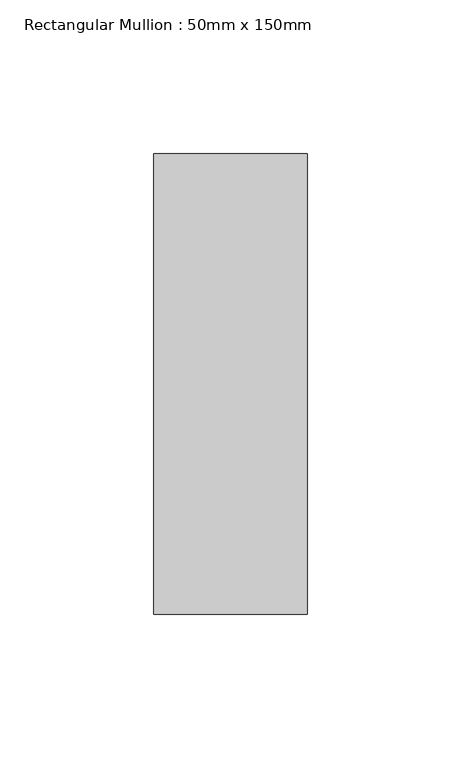
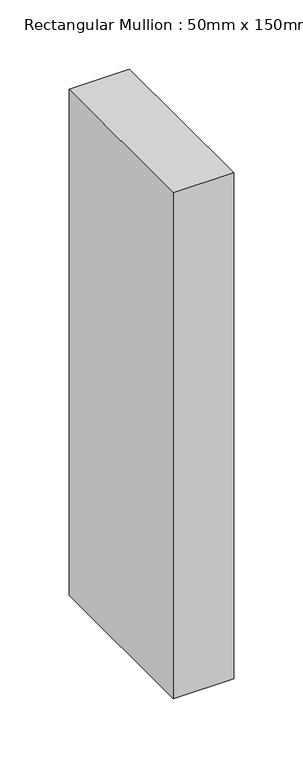
"""IFC4 building model written with IfcOpenShell, lengths in millimetres: member geometry, Rectangular Mullion : 50mm x 150mm."""

from ifc_helpers import new_model, si_unit, frame, origin, place, context, project, spatial, polyline, outline, extrude, source, transform, mapped, element, save


def rectangular_mullion_50mm_x_150mm_ffb0b627(model_context):
    return source(origin(), model_context, "Body", "SweptSolid", [
        extrude(outline(polyline([(0.0, 75.0), (0.0, -75.0), (-50.0, -75.0), (-50.0, 75.0), (0.0, 75.0)])), frame((0.0, 0.0, -445.0443662), z_axis=(0.0, 0.0, 1.0), x_axis=(1.0, 0.0, 0.0)), (0.0, 0.0, 1.0), 445.0443662),
    ])


if __name__ == "__main__":
    model = new_model("IFC4")
    model_context = context("Model", 3, world=origin())
    ifc_project = project(units=[si_unit("LENGTHUNIT", "METRE", prefix="MILLI")], contexts=[model_context])
    site = spatial("IfcSite", under=ifc_project)
    building = spatial("IfcBuilding", under=site)
    placement = place(None, origin())
    rectangular_mullion_50mm_x_150mm_shape = rectangular_mullion_50mm_x_150mm_ffb0b627(model_context)
    element("IfcMember", 1, ObjectType="Rectangular Mullion : 50mm x 150mm", at=placement, inside=building, context=model_context, shape_type="MappedRepresentation", body=[
        mapped(rectangular_mullion_50mm_x_150mm_shape, transform((0.0, 0.0, 0.0), x_axis=(1.0, 0.0, 0.0), y_axis=(0.0, 1.0, 0.0), z_axis=(0.0, 0.0, 1.0))),
    ])
    save(model, "model.ifc")

# Revit data of these elements
# Type "Rectangular Mullion : 50mm x 150mm"
#   built-in parameter 1007304 = 0.492126 (stored number, unit not read)
#   built-in parameter 1007301 = 0.082021 (stored number, unit not read)
#   built-in parameter 1007300 = 0.082021 (stored number, unit not read)
# Element 1 (IfcMember, "Rectangular Mullion : 50mm x 150mm")
#   Materials on its faces: "Aluminum"
# Materials
#   "Aluminum": class "Metal", colour RGB 247 247 247, transparency 0, Description = "Aluminum 6061", Cost = 0
